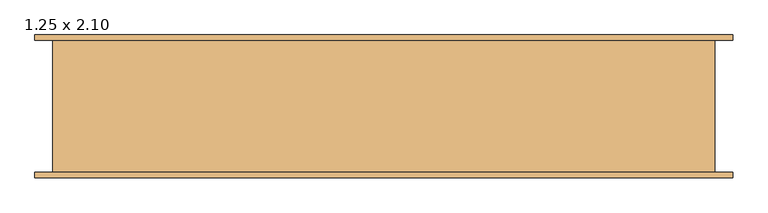
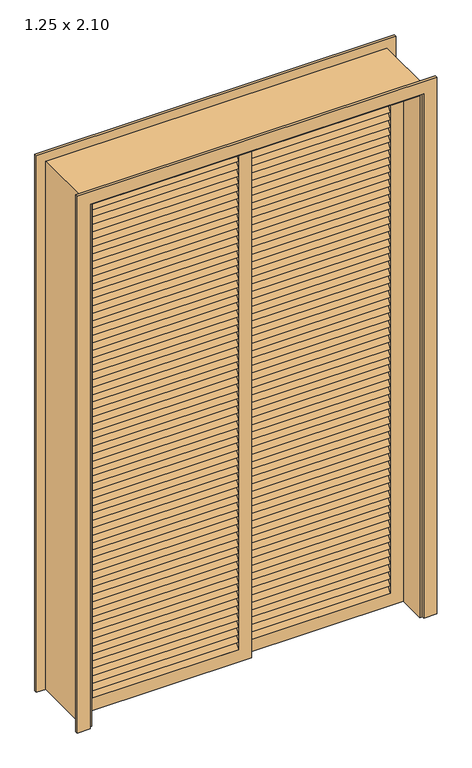
"""IFC4 building model written with IfcOpenShell, lengths in millimetres: door geometry, .CC_ND 300_PORTA DE CORRER_3 FOLHAS_VENEZIANA_VIDRO_COM EXTENSÃO : 1.25 x 2.10."""

import ifcopenshell
import ifcopenshell.guid

model = None  # the IFC model being written
_history = None  # IfcOwnerHistory: only IFC2X3 demands one
_inside = {}  # id of a spatial element -> (the spatial element, [elements in it])
_under = {}  # id of a project, library or spatial element -> (it, [spatial elements below it])
_declared = {}  # id of a project -> (the project, [libraries it declares])
_typed = {}  # id of a type object -> (the type object, [elements of that type])
_made_of = {}  # id of a material, layer set ... -> (it, [elements and type objects made of it])


def new_model(schema):
    """Start an empty IFC model of exactly this schema.

    Asked for "IFC4X3", IfcOpenShell would pick the latest addendum, in which some entities
    have other attributes; the version numbers below select the first issue.
    IFC2X3 requires an IfcOwnerHistory on every rooted entity: one is made here for all.
    """
    global model, _history
    if schema == "IFC4X3":
        model = ifcopenshell.file(schema_version=(4, 3, 0, 0))
    else:
        model = ifcopenshell.file(schema=schema)
    _inside.clear()
    _under.clear()
    _declared.clear()
    _typed.clear()
    _made_of.clear()
    _history = None
    if model.schema == "IFC2X3":
        org = make("IfcOrganization", Name="unknown")
        user = make(
            "IfcPersonAndOrganization",
            ThePerson=make("IfcPerson", FamilyName="unknown"),
            TheOrganization=org,
        )
        app = make(
            "IfcApplication",
            ApplicationDeveloper=org,
            Version="unknown",
            ApplicationFullName="unknown",
            ApplicationIdentifier="unknown",
        )
        _history = make(
            "IfcOwnerHistory",
            OwningUser=user,
            OwningApplication=app,
            ChangeAction="ADDED",
            CreationDate=0,
        )
    return model


def make(cls, **values):
    """One entity of the class cls with the attributes given. An attribute that is None is left unset."""
    return model.create_entity(
        cls, **{name: value for name, value in values.items() if value is not None}
    )


def rooted(cls, **values):
    """An entity with a GlobalId (a new one), such as an element, a storey or a relation."""
    return make(cls, GlobalId=ifcopenshell.guid.new(), OwnerHistory=_history, **values)


def si_unit(unit_type, name, prefix=None):
    """IfcSIUnit, for example si_unit("LENGTHUNIT", "METRE", prefix="MILLI")."""
    return make("IfcSIUnit", UnitType=unit_type, Prefix=prefix, Name=name)


def assignment(units):
    """IfcUnitAssignment: the units of a project."""
    return None if units is None else make("IfcUnitAssignment", Units=units)


def point(xyz):
    """IfcCartesianPoint."""
    return None if xyz is None else make("IfcCartesianPoint", Coordinates=xyz)


def direction(xyz):
    """IfcDirection."""
    return None if xyz is None else make("IfcDirection", DirectionRatios=xyz)


def frame(location, z_axis=None, x_axis=None):
    """IfcAxis2Placement3D, a coordinate frame: its origin and axes. An axis left out is left unset."""
    return make(
        "IfcAxis2Placement3D",
        Location=point(location),
        Axis=direction(z_axis),
        RefDirection=direction(x_axis),
    )


def origin():
    """The frame at (0, 0, 0) with its axes left unset."""
    return frame((0.0, 0.0, 0.0))


def place(relative_to, where):
    """IfcLocalPlacement: puts the frame where relative to a parent placement (None: the world)."""
    return make(
        "IfcLocalPlacement", PlacementRelTo=relative_to, RelativePlacement=where
    )


def context(
    kind, dimensions, precision=None, world=None, true_north=None, identifier=None
):
    """IfcGeometricRepresentationContext, for example the 3D "Model" context."""
    return make(
        "IfcGeometricRepresentationContext",
        ContextIdentifier=identifier,
        ContextType=kind,
        CoordinateSpaceDimension=dimensions,
        Precision=precision,
        WorldCoordinateSystem=world,
        TrueNorth=true_north,
    )


def project(units=None, contexts=None):
    """IfcProject with its units and contexts."""
    return rooted(
        "IfcProject",
        Name="project",
        RepresentationContexts=contexts,
        UnitsInContext=assignment(units),
    )


def spatial(cls, under=None, at=None, **own):
    """A site, building, storey or space (cls), placed at a placement, below another one or the project."""
    s = rooted(cls, ObjectPlacement=at, **own)
    if under is not None:
        _under.setdefault(under.id(), (under, []))[1].append(s)
    return s


def polyline(points):
    """IfcPolyline through the points."""
    return make("IfcPolyline", Points=[point(p) for p in points])


def outline(outer, holes=None, kind="AREA"):
    """IfcArbitraryClosedProfileDef: a profile drawn as a closed curve; with holes, ...WithVoids."""
    if holes is None:
        return make("IfcArbitraryClosedProfileDef", ProfileType=kind, OuterCurve=outer)
    return make(
        "IfcArbitraryProfileDefWithVoids",
        ProfileType=kind,
        OuterCurve=outer,
        InnerCurves=holes,
    )


def extrude(swept, where, along, depth):
    """IfcExtrudedAreaSolid: the profile swept, set in the frame where, extruded along a direction by depth."""
    return make(
        "IfcExtrudedAreaSolid",
        SweptArea=swept,
        Position=where,
        ExtrudedDirection=direction(along),
        Depth=depth,
    )


def shape(context_of_items, identifier, shape_type, items):
    """IfcShapeRepresentation: the items that make up one representation, for example the "Body"."""
    return make(
        "IfcShapeRepresentation",
        ContextOfItems=context_of_items,
        RepresentationIdentifier=identifier,
        RepresentationType=shape_type,
        Items=items,
    )


def source(mapping_origin, context_of_items, identifier, shape_type, items):
    """IfcRepresentationMap: a shape defined once, which mapped items show again and again."""
    return make(
        "IfcRepresentationMap",
        MappingOrigin=mapping_origin,
        MappedRepresentation=shape(context_of_items, identifier, shape_type, items),
    )


def transform(
    local_origin,
    x_axis=None,
    y_axis=None,
    z_axis=None,
    scale=None,
    scale2=None,
    scale3=None,
    uniform=True,
):
    """IfcCartesianTransformationOperator3D, or its non-uniform kind. x_axis, y_axis, z_axis: its Axis1, 2, 3."""
    if uniform:
        return make(
            "IfcCartesianTransformationOperator3D",
            Axis1=direction(x_axis),
            Axis2=direction(y_axis),
            LocalOrigin=point(local_origin),
            Scale=scale,
            Axis3=direction(z_axis),
        )
    return make(
        "IfcCartesianTransformationOperator3DnonUniform",
        Axis1=direction(x_axis),
        Axis2=direction(y_axis),
        LocalOrigin=point(local_origin),
        Scale=scale,
        Axis3=direction(z_axis),
        Scale2=scale2,
        Scale3=scale3,
    )


def mapped(mapping_source, mapping_target):
    """IfcMappedItem: shows the shape of a source again, moved by a transform."""
    return make(
        "IfcMappedItem", MappingSource=mapping_source, MappingTarget=mapping_target
    )


def made_of(thing, what):
    """Note that an element or type object is made of a material, layer set ...; save() writes the relation."""
    if what is not None:
        _made_of.setdefault(what.id(), (what, []))[1].append(thing)
    return thing


def element(
    cls,
    number,
    at=None,
    inside=None,
    cuts=None,
    type_object=None,
    material=None,
    context=None,
    identifier="Body",
    shape_type=None,
    held_by="IfcProductDefinitionShape",
    body=None,
    shapes=None,
    **own,
):
    """One element of the class cls, such as IfcWall. Its Tag is "e" and its number.

    at: its placement. inside: the storey or other place that contains it. cuts: it is an
    opening in that element (IfcRelVoidsElement). A single representation is given by context,
    identifier, shape_type and body (its items); several are given by shapes. held_by: the class
    of the entity that holds the representations. save() writes the other relations.
    """
    e = rooted(cls, Tag="e%d" % number, ObjectPlacement=at, **own)
    if body is not None:
        shapes = [shape(context, identifier, shape_type, body)]
    if shapes is not None:
        e.Representation = make(held_by, Representations=shapes)
    if inside is not None:
        _inside.setdefault(inside.id(), (inside, []))[1].append(e)
    if cuts is not None:
        rooted(
            "IfcRelVoidsElement", RelatingBuildingElement=cuts, RelatedOpeningElement=e
        )
    if type_object is not None:
        _typed.setdefault(type_object.id(), (type_object, []))[1].append(e)
    return made_of(e, material)


def aggregate(whole, parts):
    """IfcRelAggregates: a whole, such as a stair, and the parts it consists of."""
    return rooted("IfcRelAggregates", RelatingObject=whole, RelatedObjects=parts)


def save(model, path):
    """Write the relations noted so far, then the file.

    IfcRelAggregates (storeys below a building ...), IfcRelContainedInSpatialStructure (elements
    in a storey), IfcRelDefinesByType, IfcRelAssociatesMaterial and IfcRelDeclares: one each for
    every whole, place, type object, material and project.
    """
    for whole, parts in _under.values():
        aggregate(whole, parts)
    for where, things in _inside.values():
        rooted(
            "IfcRelContainedInSpatialStructure",
            RelatedElements=things,
            RelatingStructure=where,
        )
    for kind, things in _typed.values():
        rooted("IfcRelDefinesByType", RelatedObjects=things, RelatingType=kind)
    for what, things in _made_of.values():
        rooted("IfcRelAssociatesMaterial", RelatedObjects=things, RelatingMaterial=what)
    for by, libraries in _declared.values():
        rooted("IfcRelDeclares", RelatingContext=by, RelatedDefinitions=libraries)
    model.write(path)


def door_1_25_x_2_10_052434fb(model_context):
    return source(origin(), model_context, "Body", "SweptSolid", [
        extrude(outline(polyline([(575.0, 26.0), (20.0, 26.0), (20.0, 34.0), (575.0, 34.0), (575.0, 26.0)])), frame((0.0, 0.0, 50.0), z_axis=(0.0, 0.0, 1.0), x_axis=(1.0, 0.0, 0.0)), (0.0, 0.0, 1.0), 2000.0),
        extrude(outline(polyline([(2100.0, 625.0), (2100.0, -30.0), (0.0, -30.0), (0.0, 625.0), (2100.0, 625.0)]), holes=[polyline([(2050.0, 575.0), (50.0, 575.0), (50.0, 20.0), (2050.0, 20.0), (2050.0, 575.0)])]), frame((0.0, 15.0, 0.0), z_axis=(0.0, 1.0, 0.0), x_axis=(0.0, 0.0, 1.0)), (0.0, 0.0, 1.0), 30.0),
        extrude(outline(polyline([(-40.0, 1985.2272727), (-45.0, 1985.2272727), (-20.0, 2020.2272727), (-15.0, 2020.2272727), (-40.0, 1985.2272727)])), frame((-575.0, 0.0, 0.0), z_axis=(1.0, 0.0, 0.0), x_axis=(0.0, 1.0, 0.0)), (0.0, 0.0, 1.0), 555.0),
        extrude(outline(polyline([(-40.0, 1955.4545455), (-45.0, 1955.4545455), (-20.0, 1990.4545455), (-15.0, 1990.4545455), (-40.0, 1955.4545455)])), frame((-575.0, 0.0, 0.0), z_axis=(1.0, 0.0, 0.0), x_axis=(0.0, 1.0, 0.0)), (0.0, 0.0, 1.0), 555.0),
        extrude(outline(polyline([(-40.0, 1925.6818182), (-45.0, 1925.6818182), (-20.0, 1960.6818182), (-15.0, 1960.6818182), (-40.0, 1925.6818182)])), frame((-575.0, 0.0, 0.0), z_axis=(1.0, 0.0, 0.0), x_axis=(0.0, 1.0, 0.0)), (0.0, 0.0, 1.0), 555.0),
        extrude(outline(polyline([(-40.0, 1895.9090909), (-45.0, 1895.9090909), (-20.0, 1930.9090909), (-15.0, 1930.9090909), (-40.0, 1895.9090909)])), frame((-575.0, 0.0, 0.0), z_axis=(1.0, 0.0, 0.0), x_axis=(0.0, 1.0, 0.0)), (0.0, 0.0, 1.0), 555.0),
        extrude(outline(polyline([(-40.0, 1866.1363636), (-45.0, 1866.1363636), (-20.0, 1901.1363636), (-15.0, 1901.1363636), (-40.0, 1866.1363636)])), frame((-575.0, 0.0, 0.0), z_axis=(1.0, 0.0, 0.0), x_axis=(0.0, 1.0, 0.0)), (0.0, 0.0, 1.0), 555.0),
        extrude(outline(polyline([(-40.0, 1836.3636364), (-45.0, 1836.3636364), (-20.0, 1871.3636364), (-15.0, 1871.3636364), (-40.0, 1836.3636364)])), frame((-575.0, 0.0, 0.0), z_axis=(1.0, 0.0, 0.0), x_axis=(0.0, 1.0, 0.0)), (0.0, 0.0, 1.0), 555.0),
        extrude(outline(polyline([(-40.0, 1806.5909091), (-45.0, 1806.5909091), (-20.0, 1841.5909091), (-15.0, 1841.5909091), (-40.0, 1806.5909091)])), frame((-575.0, 0.0, 0.0), z_axis=(1.0, 0.0, 0.0), x_axis=(0.0, 1.0, 0.0)), (0.0, 0.0, 1.0), 555.0),
        extrude(outline(polyline([(-40.0, 1776.8181818), (-45.0, 1776.8181818), (-20.0, 1811.8181818), (-15.0, 1811.8181818), (-40.0, 1776.8181818)])), frame((-575.0, 0.0, 0.0), z_axis=(1.0, 0.0, 0.0), x_axis=(0.0, 1.0, 0.0)), (0.0, 0.0, 1.0), 555.0),
        extrude(outline(polyline([(-40.0, 1747.0454545), (-45.0, 1747.0454545), (-20.0, 1782.0454545), (-15.0, 1782.0454545), (-40.0, 1747.0454545)])), frame((-575.0, 0.0, 0.0), z_axis=(1.0, 0.0, 0.0), x_axis=(0.0, 1.0, 0.0)), (0.0, 0.0, 1.0), 555.0),
        extrude(outline(polyline([(-40.0, 1717.2727273), (-45.0, 1717.2727273), (-20.0, 1752.2727273), (-15.0, 1752.2727273), (-40.0, 1717.2727273)])), frame((-575.0, 0.0, 0.0), z_axis=(1.0, 0.0, 0.0), x_axis=(0.0, 1.0, 0.0)), (0.0, 0.0, 1.0), 555.0),
        extrude(outline(polyline([(-40.0, 1687.5), (-45.0, 1687.5), (-20.0, 1722.5), (-15.0, 1722.5), (-40.0, 1687.5)])), frame((-575.0, 0.0, 0.0), z_axis=(1.0, 0.0, 0.0), x_axis=(0.0, 1.0, 0.0)), (0.0, 0.0, 1.0), 555.0),
        extrude(outline(polyline([(-40.0, 1657.7272727), (-45.0, 1657.7272727), (-20.0, 1692.7272727), (-15.0, 1692.7272727), (-40.0, 1657.7272727)])), frame((-575.0, 0.0, 0.0), z_axis=(1.0, 0.0, 0.0), x_axis=(0.0, 1.0, 0.0)), (0.0, 0.0, 1.0), 555.0),
        extrude(outline(polyline([(-40.0, 1627.9545455), (-45.0, 1627.9545455), (-20.0, 1662.9545455), (-15.0, 1662.9545455), (-40.0, 1627.9545455)])), frame((-575.0, 0.0, 0.0), z_axis=(1.0, 0.0, 0.0), x_axis=(0.0, 1.0, 0.0)), (0.0, 0.0, 1.0), 555.0),
        extrude(outline(polyline([(-40.0, 1598.1818182), (-45.0, 1598.1818182), (-20.0, 1633.1818182), (-15.0, 1633.1818182), (-40.0, 1598.1818182)])), frame((-575.0, 0.0, 0.0), z_axis=(1.0, 0.0, 0.0), x_axis=(0.0, 1.0, 0.0)), (0.0, 0.0, 1.0), 555.0),
        extrude(outline(polyline([(-40.0, 1568.4090909), (-45.0, 1568.4090909), (-20.0, 1603.4090909), (-15.0, 1603.4090909), (-40.0, 1568.4090909)])), frame((-575.0, 0.0, 0.0), z_axis=(1.0, 0.0, 0.0), x_axis=(0.0, 1.0, 0.0)), (0.0, 0.0, 1.0), 555.0),
        extrude(outline(polyline([(-40.0, 1538.6363636), (-45.0, 1538.6363636), (-20.0, 1573.6363636), (-15.0, 1573.6363636), (-40.0, 1538.6363636)])), frame((-575.0, 0.0, 0.0), z_axis=(1.0, 0.0, 0.0), x_axis=(0.0, 1.0, 0.0)), (0.0, 0.0, 1.0), 555.0),
        extrude(outline(polyline([(-40.0, 1508.8636364), (-45.0, 1508.8636364), (-20.0, 1543.8636364), (-15.0, 1543.8636364), (-40.0, 1508.8636364)])), frame((-575.0, 0.0, 0.0), z_axis=(1.0, 0.0, 0.0), x_axis=(0.0, 1.0, 0.0)), (0.0, 0.0, 1.0), 555.0),
        extrude(outline(polyline([(-40.0, 1479.0909091), (-45.0, 1479.0909091), (-20.0, 1514.0909091), (-15.0, 1514.0909091), (-40.0, 1479.0909091)])), frame((-575.0, 0.0, 0.0), z_axis=(1.0, 0.0, 0.0), x_axis=(0.0, 1.0, 0.0)), (0.0, 0.0, 1.0), 555.0),
        extrude(outline(polyline([(-40.0, 1449.3181818), (-45.0, 1449.3181818), (-20.0, 1484.3181818), (-15.0, 1484.3181818), (-40.0, 1449.3181818)])), frame((-575.0, 0.0, 0.0), z_axis=(1.0, 0.0, 0.0), x_axis=(0.0, 1.0, 0.0)), (0.0, 0.0, 1.0), 555.0),
        extrude(outline(polyline([(-40.0, 1419.5454545), (-45.0, 1419.5454545), (-20.0, 1454.5454545), (-15.0, 1454.5454545), (-40.0, 1419.5454545)])), frame((-575.0, 0.0, 0.0), z_axis=(1.0, 0.0, 0.0), x_axis=(0.0, 1.0, 0.0)), (0.0, 0.0, 1.0), 555.0),
        extrude(outline(polyline([(-40.0, 1389.7727273), (-45.0, 1389.7727273), (-20.0, 1424.7727273), (-15.0, 1424.7727273), (-40.0, 1389.7727273)])), frame((-575.0, 0.0, 0.0), z_axis=(1.0, 0.0, 0.0), x_axis=(0.0, 1.0, 0.0)), (0.0, 0.0, 1.0), 555.0),
        extrude(outline(polyline([(-40.0, 1360.0), (-45.0, 1360.0), (-20.0, 1395.0), (-15.0, 1395.0), (-40.0, 1360.0)])), frame((-575.0, 0.0, 0.0), z_axis=(1.0, 0.0, 0.0), x_axis=(0.0, 1.0, 0.0)), (0.0, 0.0, 1.0), 555.0),
        extrude(outline(polyline([(-40.0, 1330.2272727), (-45.0, 1330.2272727), (-20.0, 1365.2272727), (-15.0, 1365.2272727), (-40.0, 1330.2272727)])), frame((-575.0, 0.0, 0.0), z_axis=(1.0, 0.0, 0.0), x_axis=(0.0, 1.0, 0.0)), (0.0, 0.0, 1.0), 555.0),
        extrude(outline(polyline([(-40.0, 1300.4545455), (-45.0, 1300.4545455), (-20.0, 1335.4545455), (-15.0, 1335.4545455), (-40.0, 1300.4545455)])), frame((-575.0, 0.0, 0.0), z_axis=(1.0, 0.0, 0.0), x_axis=(0.0, 1.0, 0.0)), (0.0, 0.0, 1.0), 555.0),
        extrude(outline(polyline([(-40.0, 1270.6818182), (-45.0, 1270.6818182), (-20.0, 1305.6818182), (-15.0, 1305.6818182), (-40.0, 1270.6818182)])), frame((-575.0, 0.0, 0.0), z_axis=(1.0, 0.0, 0.0), x_axis=(0.0, 1.0, 0.0)), (0.0, 0.0, 1.0), 555.0),
        extrude(outline(polyline([(-40.0, 1240.9090909), (-45.0, 1240.9090909), (-20.0, 1275.9090909), (-15.0, 1275.9090909), (-40.0, 1240.9090909)])), frame((-575.0, 0.0, 0.0), z_axis=(1.0, 0.0, 0.0), x_axis=(0.0, 1.0, 0.0)), (0.0, 0.0, 1.0), 555.0),
        extrude(outline(polyline([(-40.0, 1211.1363636), (-45.0, 1211.1363636), (-20.0, 1246.1363636), (-15.0, 1246.1363636), (-40.0, 1211.1363636)])), frame((-575.0, 0.0, 0.0), z_axis=(1.0, 0.0, 0.0), x_axis=(0.0, 1.0, 0.0)), (0.0, 0.0, 1.0), 555.0),
        extrude(outline(polyline([(-40.0, 1181.3636364), (-45.0, 1181.3636364), (-20.0, 1216.3636364), (-15.0, 1216.3636364), (-40.0, 1181.3636364)])), frame((-575.0, 0.0, 0.0), z_axis=(1.0, 0.0, 0.0), x_axis=(0.0, 1.0, 0.0)), (0.0, 0.0, 1.0), 555.0),
        extrude(outline(polyline([(-40.0, 1151.5909091), (-45.0, 1151.5909091), (-20.0, 1186.5909091), (-15.0, 1186.5909091), (-40.0, 1151.5909091)])), frame((-575.0, 0.0, 0.0), z_axis=(1.0, 0.0, 0.0), x_axis=(0.0, 1.0, 0.0)), (0.0, 0.0, 1.0), 555.0),
        extrude(outline(polyline([(-40.0, 1121.8181818), (-45.0, 1121.8181818), (-20.0, 1156.8181818), (-15.0, 1156.8181818), (-40.0, 1121.8181818)])), frame((-575.0, 0.0, 0.0), z_axis=(1.0, 0.0, 0.0), x_axis=(0.0, 1.0, 0.0)), (0.0, 0.0, 1.0), 555.0),
        extrude(outline(polyline([(-40.0, 1092.0454545), (-45.0, 1092.0454545), (-20.0, 1127.0454545), (-15.0, 1127.0454545), (-40.0, 1092.0454545)])), frame((-575.0, 0.0, 0.0), z_axis=(1.0, 0.0, 0.0), x_axis=(0.0, 1.0, 0.0)), (0.0, 0.0, 1.0), 555.0),
        extrude(outline(polyline([(-40.0, 1062.2727273), (-45.0, 1062.2727273), (-20.0, 1097.2727273), (-15.0, 1097.2727273), (-40.0, 1062.2727273)])), frame((-575.0, 0.0, 0.0), z_axis=(1.0, 0.0, 0.0), x_axis=(0.0, 1.0, 0.0)), (0.0, 0.0, 1.0), 555.0),
        extrude(outline(polyline([(-40.0, 1032.5), (-45.0, 1032.5), (-20.0, 1067.5), (-15.0, 1067.5), (-40.0, 1032.5)])), frame((-575.0, 0.0, 0.0), z_axis=(1.0, 0.0, 0.0), x_axis=(0.0, 1.0, 0.0)), (0.0, 0.0, 1.0), 555.0),
        extrude(outline(polyline([(-40.0, 1002.7272727), (-45.0, 1002.7272727), (-20.0, 1037.7272727), (-15.0, 1037.7272727), (-40.0, 1002.7272727)])), frame((-575.0, 0.0, 0.0), z_axis=(1.0, 0.0, 0.0), x_axis=(0.0, 1.0, 0.0)), (0.0, 0.0, 1.0), 555.0),
        extrude(outline(polyline([(-40.0, 972.9545455), (-45.0, 972.9545455), (-20.0, 1007.9545455), (-15.0, 1007.9545455), (-40.0, 972.9545455)])), frame((-575.0, 0.0, 0.0), z_axis=(1.0, 0.0, 0.0), x_axis=(0.0, 1.0, 0.0)), (0.0, 0.0, 1.0), 555.0),
        extrude(outline(polyline([(-40.0, 943.1818182), (-45.0, 943.1818182), (-20.0, 978.1818182), (-15.0, 978.1818182), (-40.0, 943.1818182)])), frame((-575.0, 0.0, 0.0), z_axis=(1.0, 0.0, 0.0), x_axis=(0.0, 1.0, 0.0)), (0.0, 0.0, 1.0), 555.0),
        extrude(outline(polyline([(-40.0, 913.4090909), (-45.0, 913.4090909), (-20.0, 948.4090909), (-15.0, 948.4090909), (-40.0, 913.4090909)])), frame((-575.0, 0.0, 0.0), z_axis=(1.0, 0.0, 0.0), x_axis=(0.0, 1.0, 0.0)), (0.0, 0.0, 1.0), 555.0),
        extrude(outline(polyline([(-40.0, 883.6363636), (-45.0, 883.6363636), (-20.0, 918.6363636), (-15.0, 918.6363636), (-40.0, 883.6363636)])), frame((-575.0, 0.0, 0.0), z_axis=(1.0, 0.0, 0.0), x_axis=(0.0, 1.0, 0.0)), (0.0, 0.0, 1.0), 555.0),
        extrude(outline(polyline([(-40.0, 853.8636364), (-45.0, 853.8636364), (-20.0, 888.8636364), (-15.0, 888.8636364), (-40.0, 853.8636364)])), frame((-575.0, 0.0, 0.0), z_axis=(1.0, 0.0, 0.0), x_axis=(0.0, 1.0, 0.0)), (0.0, 0.0, 1.0), 555.0),
        extrude(outline(polyline([(-40.0, 824.0909091), (-45.0, 824.0909091), (-20.0, 859.0909091), (-15.0, 859.0909091), (-40.0, 824.0909091)])), frame((-575.0, 0.0, 0.0), z_axis=(1.0, 0.0, 0.0), x_axis=(0.0, 1.0, 0.0)), (0.0, 0.0, 1.0), 555.0),
        extrude(outline(polyline([(-40.0, 794.3181818), (-45.0, 794.3181818), (-20.0, 829.3181818), (-15.0, 829.3181818), (-40.0, 794.3181818)])), frame((-575.0, 0.0, 0.0), z_axis=(1.0, 0.0, 0.0), x_axis=(0.0, 1.0, 0.0)), (0.0, 0.0, 1.0), 555.0),
        extrude(outline(polyline([(-40.0, 764.5454545), (-45.0, 764.5454545), (-20.0, 799.5454545), (-15.0, 799.5454545), (-40.0, 764.5454545)])), frame((-575.0, 0.0, 0.0), z_axis=(1.0, 0.0, 0.0), x_axis=(0.0, 1.0, 0.0)), (0.0, 0.0, 1.0), 555.0),
        extrude(outline(polyline([(-40.0, 734.7727273), (-45.0, 734.7727273), (-20.0, 769.7727273), (-15.0, 769.7727273), (-40.0, 734.7727273)])), frame((-575.0, 0.0, 0.0), z_axis=(1.0, 0.0, 0.0), x_axis=(0.0, 1.0, 0.0)), (0.0, 0.0, 1.0), 555.0),
        extrude(outline(polyline([(-40.0, 705.0), (-45.0, 705.0), (-20.0, 740.0), (-15.0, 740.0), (-40.0, 705.0)])), frame((-575.0, 0.0, 0.0), z_axis=(1.0, 0.0, 0.0), x_axis=(0.0, 1.0, 0.0)), (0.0, 0.0, 1.0), 555.0),
        extrude(outline(polyline([(-40.0, 675.2272727), (-45.0, 675.2272727), (-20.0, 710.2272727), (-15.0, 710.2272727), (-40.0, 675.2272727)])), frame((-575.0, 0.0, 0.0), z_axis=(1.0, 0.0, 0.0), x_axis=(0.0, 1.0, 0.0)), (0.0, 0.0, 1.0), 555.0),
        extrude(outline(polyline([(-40.0, 645.4545455), (-45.0, 645.4545455), (-20.0, 680.4545455), (-15.0, 680.4545455), (-40.0, 645.4545455)])), frame((-575.0, 0.0, 0.0), z_axis=(1.0, 0.0, 0.0), x_axis=(0.0, 1.0, 0.0)), (0.0, 0.0, 1.0), 555.0),
        extrude(outline(polyline([(-40.0, 615.6818182), (-45.0, 615.6818182), (-20.0, 650.6818182), (-15.0, 650.6818182), (-40.0, 615.6818182)])), frame((-575.0, 0.0, 0.0), z_axis=(1.0, 0.0, 0.0), x_axis=(0.0, 1.0, 0.0)), (0.0, 0.0, 1.0), 555.0),
        extrude(outline(polyline([(-40.0, 585.9090909), (-45.0, 585.9090909), (-20.0, 620.9090909), (-15.0, 620.9090909), (-40.0, 585.9090909)])), frame((-575.0, 0.0, 0.0), z_axis=(1.0, 0.0, 0.0), x_axis=(0.0, 1.0, 0.0)), (0.0, 0.0, 1.0), 555.0),
        extrude(outline(polyline([(-40.0, 556.1363636), (-45.0, 556.1363636), (-20.0, 591.1363636), (-15.0, 591.1363636), (-40.0, 556.1363636)])), frame((-575.0, 0.0, 0.0), z_axis=(1.0, 0.0, 0.0), x_axis=(0.0, 1.0, 0.0)), (0.0, 0.0, 1.0), 555.0),
        extrude(outline(polyline([(-40.0, 526.3636364), (-45.0, 526.3636364), (-20.0, 561.3636364), (-15.0, 561.3636364), (-40.0, 526.3636364)])), frame((-575.0, 0.0, 0.0), z_axis=(1.0, 0.0, 0.0), x_axis=(0.0, 1.0, 0.0)), (0.0, 0.0, 1.0), 555.0),
        extrude(outline(polyline([(-40.0, 496.5909091), (-45.0, 496.5909091), (-20.0, 531.5909091), (-15.0, 531.5909091), (-40.0, 496.5909091)])), frame((-575.0, 0.0, 0.0), z_axis=(1.0, 0.0, 0.0), x_axis=(0.0, 1.0, 0.0)), (0.0, 0.0, 1.0), 555.0),
        extrude(outline(polyline([(-40.0, 466.8181818), (-45.0, 466.8181818), (-20.0, 501.8181818), (-15.0, 501.8181818), (-40.0, 466.8181818)])), frame((-575.0, 0.0, 0.0), z_axis=(1.0, 0.0, 0.0), x_axis=(0.0, 1.0, 0.0)), (0.0, 0.0, 1.0), 555.0),
        extrude(outline(polyline([(-40.0, 437.0454545), (-45.0, 437.0454545), (-20.0, 472.0454545), (-15.0, 472.0454545), (-40.0, 437.0454545)])), frame((-575.0, 0.0, 0.0), z_axis=(1.0, 0.0, 0.0), x_axis=(0.0, 1.0, 0.0)), (0.0, 0.0, 1.0), 555.0),
        extrude(outline(polyline([(-40.0, 407.2727273), (-45.0, 407.2727273), (-20.0, 442.2727273), (-15.0, 442.2727273), (-40.0, 407.2727273)])), frame((-575.0, 0.0, 0.0), z_axis=(1.0, 0.0, 0.0), x_axis=(0.0, 1.0, 0.0)), (0.0, 0.0, 1.0), 555.0),
        extrude(outline(polyline([(-40.0, 377.5), (-45.0, 377.5), (-20.0, 412.5), (-15.0, 412.5), (-40.0, 377.5)])), frame((-575.0, 0.0, 0.0), z_axis=(1.0, 0.0, 0.0), x_axis=(0.0, 1.0, 0.0)), (0.0, 0.0, 1.0), 555.0),
        extrude(outline(polyline([(-40.0, 347.7272727), (-45.0, 347.7272727), (-20.0, 382.7272727), (-15.0, 382.7272727), (-40.0, 347.7272727)])), frame((-575.0, 0.0, 0.0), z_axis=(1.0, 0.0, 0.0), x_axis=(0.0, 1.0, 0.0)), (0.0, 0.0, 1.0), 555.0),
        extrude(outline(polyline([(-40.0, 317.9545455), (-45.0, 317.9545455), (-20.0, 352.9545455), (-15.0, 352.9545455), (-40.0, 317.9545455)])), frame((-575.0, 0.0, 0.0), z_axis=(1.0, 0.0, 0.0), x_axis=(0.0, 1.0, 0.0)), (0.0, 0.0, 1.0), 555.0),
        extrude(outline(polyline([(-40.0, 288.1818182), (-45.0, 288.1818182), (-20.0, 323.1818182), (-15.0, 323.1818182), (-40.0, 288.1818182)])), frame((-575.0, 0.0, 0.0), z_axis=(1.0, 0.0, 0.0), x_axis=(0.0, 1.0, 0.0)), (0.0, 0.0, 1.0), 555.0),
        extrude(outline(polyline([(-40.0, 258.4090909), (-45.0, 258.4090909), (-20.0, 293.4090909), (-15.0, 293.4090909), (-40.0, 258.4090909)])), frame((-575.0, 0.0, 0.0), z_axis=(1.0, 0.0, 0.0), x_axis=(0.0, 1.0, 0.0)), (0.0, 0.0, 1.0), 555.0),
        extrude(outline(polyline([(-40.0, 228.6363636), (-45.0, 228.6363636), (-20.0, 263.6363636), (-15.0, 263.6363636), (-40.0, 228.6363636)])), frame((-575.0, 0.0, 0.0), z_axis=(1.0, 0.0, 0.0), x_axis=(0.0, 1.0, 0.0)), (0.0, 0.0, 1.0), 555.0),
        extrude(outline(polyline([(-40.0, 198.8636364), (-45.0, 198.8636364), (-20.0, 233.8636364), (-15.0, 233.8636364), (-40.0, 198.8636364)])), frame((-575.0, 0.0, 0.0), z_axis=(1.0, 0.0, 0.0), x_axis=(0.0, 1.0, 0.0)), (0.0, 0.0, 1.0), 555.0),
        extrude(outline(polyline([(-40.0, 169.0909091), (-45.0, 169.0909091), (-20.0, 204.0909091), (-15.0, 204.0909091), (-40.0, 169.0909091)])), frame((-575.0, 0.0, 0.0), z_axis=(1.0, 0.0, 0.0), x_axis=(0.0, 1.0, 0.0)), (0.0, 0.0, 1.0), 555.0),
        extrude(outline(polyline([(-40.0, 139.3181818), (-45.0, 139.3181818), (-20.0, 174.3181818), (-15.0, 174.3181818), (-40.0, 139.3181818)])), frame((-575.0, 0.0, 0.0), z_axis=(1.0, 0.0, 0.0), x_axis=(0.0, 1.0, 0.0)), (0.0, 0.0, 1.0), 555.0),
        extrude(outline(polyline([(-40.0, 109.5454545), (-45.0, 109.5454545), (-20.0, 144.5454545), (-15.0, 144.5454545), (-40.0, 109.5454545)])), frame((-575.0, 0.0, 0.0), z_axis=(1.0, 0.0, 0.0), x_axis=(0.0, 1.0, 0.0)), (0.0, 0.0, 1.0), 555.0),
        extrude(outline(polyline([(-40.0, 79.7727273), (-45.0, 79.7727273), (-20.0, 114.7727273), (-15.0, 114.7727273), (-40.0, 79.7727273)])), frame((-575.0, 0.0, 0.0), z_axis=(1.0, 0.0, 0.0), x_axis=(0.0, 1.0, 0.0)), (0.0, 0.0, 1.0), 555.0),
        extrude(outline(polyline([(-40.0, 2015.0), (-45.0, 2015.0), (-20.0, 2050.0), (-15.0, 2050.0), (-40.0, 2015.0)])), frame((-575.0, 0.0, 0.0), z_axis=(1.0, 0.0, 0.0), x_axis=(0.0, 1.0, 0.0)), (0.0, 0.0, 1.0), 555.0),
        extrude(outline(polyline([(-40.0, 50.0), (-45.0, 50.0), (-20.0, 85.0), (-15.0, 85.0), (-40.0, 50.0)])), frame((-575.0, 0.0, 0.0), z_axis=(1.0, 0.0, 0.0), x_axis=(0.0, 1.0, 0.0)), (0.0, 0.0, 1.0), 555.0),
        extrude(outline(polyline([(2100.0, 30.0), (2100.0, -625.0), (0.0, -625.0), (0.0, 30.0), (2100.0, 30.0)]), holes=[polyline([(2050.0, -20.0), (50.0, -20.0), (50.0, -575.0), (2050.0, -575.0), (2050.0, -20.0)])]), frame((0.0, -45.0, 0.0), z_axis=(0.0, 1.0, 0.0), x_axis=(0.0, 0.0, 1.0)), (0.0, 0.0, 1.0), 30.0),
        extrude(outline(polyline([(-10.0, 1985.2272727), (-15.0, 1985.2272727), (10.0, 2020.2272727), (15.0, 2020.2272727), (-10.0, 1985.2272727)])), frame((20.0, 0.0, 0.0), z_axis=(1.0, 0.0, 0.0), x_axis=(0.0, 1.0, 0.0)), (0.0, 0.0, 1.0), 555.0),
        extrude(outline(polyline([(-10.0, 1955.4545455), (-15.0, 1955.4545455), (10.0, 1990.4545455), (15.0, 1990.4545455), (-10.0, 1955.4545455)])), frame((20.0, 0.0, 0.0), z_axis=(1.0, 0.0, 0.0), x_axis=(0.0, 1.0, 0.0)), (0.0, 0.0, 1.0), 555.0),
        extrude(outline(polyline([(-10.0, 1925.6818182), (-15.0, 1925.6818182), (10.0, 1960.6818182), (15.0, 1960.6818182), (-10.0, 1925.6818182)])), frame((20.0, 0.0, 0.0), z_axis=(1.0, 0.0, 0.0), x_axis=(0.0, 1.0, 0.0)), (0.0, 0.0, 1.0), 555.0),
        extrude(outline(polyline([(-10.0, 1895.9090909), (-15.0, 1895.9090909), (10.0, 1930.9090909), (15.0, 1930.9090909), (-10.0, 1895.9090909)])), frame((20.0, 0.0, 0.0), z_axis=(1.0, 0.0, 0.0), x_axis=(0.0, 1.0, 0.0)), (0.0, 0.0, 1.0), 555.0),
        extrude(outline(polyline([(-10.0, 1866.1363636), (-15.0, 1866.1363636), (10.0, 1901.1363636), (15.0, 1901.1363636), (-10.0, 1866.1363636)])), frame((20.0, 0.0, 0.0), z_axis=(1.0, 0.0, 0.0), x_axis=(0.0, 1.0, 0.0)), (0.0, 0.0, 1.0), 555.0),
        extrude(outline(polyline([(-10.0, 1836.3636364), (-15.0, 1836.3636364), (10.0, 1871.3636364), (15.0, 1871.3636364), (-10.0, 1836.3636364)])), frame((20.0, 0.0, 0.0), z_axis=(1.0, 0.0, 0.0), x_axis=(0.0, 1.0, 0.0)), (0.0, 0.0, 1.0), 555.0),
        extrude(outline(polyline([(-10.0, 1806.5909091), (-15.0, 1806.5909091), (10.0, 1841.5909091), (15.0, 1841.5909091), (-10.0, 1806.5909091)])), frame((20.0, 0.0, 0.0), z_axis=(1.0, 0.0, 0.0), x_axis=(0.0, 1.0, 0.0)), (0.0, 0.0, 1.0), 555.0),
        extrude(outline(polyline([(-10.0, 1776.8181818), (-15.0, 1776.8181818), (10.0, 1811.8181818), (15.0, 1811.8181818), (-10.0, 1776.8181818)])), frame((20.0, 0.0, 0.0), z_axis=(1.0, 0.0, 0.0), x_axis=(0.0, 1.0, 0.0)), (0.0, 0.0, 1.0), 555.0),
        extrude(outline(polyline([(-10.0, 1747.0454545), (-15.0, 1747.0454545), (10.0, 1782.0454545), (15.0, 1782.0454545), (-10.0, 1747.0454545)])), frame((20.0, 0.0, 0.0), z_axis=(1.0, 0.0, 0.0), x_axis=(0.0, 1.0, 0.0)), (0.0, 0.0, 1.0), 555.0),
        extrude(outline(polyline([(-10.0, 1717.2727273), (-15.0, 1717.2727273), (10.0, 1752.2727273), (15.0, 1752.2727273), (-10.0, 1717.2727273)])), frame((20.0, 0.0, 0.0), z_axis=(1.0, 0.0, 0.0), x_axis=(0.0, 1.0, 0.0)), (0.0, 0.0, 1.0), 555.0),
        extrude(outline(polyline([(-10.0, 1687.5), (-15.0, 1687.5), (10.0, 1722.5), (15.0, 1722.5), (-10.0, 1687.5)])), frame((20.0, 0.0, 0.0), z_axis=(1.0, 0.0, 0.0), x_axis=(0.0, 1.0, 0.0)), (0.0, 0.0, 1.0), 555.0),
        extrude(outline(polyline([(-10.0, 1657.7272727), (-15.0, 1657.7272727), (10.0, 1692.7272727), (15.0, 1692.7272727), (-10.0, 1657.7272727)])), frame((20.0, 0.0, 0.0), z_axis=(1.0, 0.0, 0.0), x_axis=(0.0, 1.0, 0.0)), (0.0, 0.0, 1.0), 555.0),
        extrude(outline(polyline([(-10.0, 1627.9545455), (-15.0, 1627.9545455), (10.0, 1662.9545455), (15.0, 1662.9545455), (-10.0, 1627.9545455)])), frame((20.0, 0.0, 0.0), z_axis=(1.0, 0.0, 0.0), x_axis=(0.0, 1.0, 0.0)), (0.0, 0.0, 1.0), 555.0),
        extrude(outline(polyline([(-10.0, 1598.1818182), (-15.0, 1598.1818182), (10.0, 1633.1818182), (15.0, 1633.1818182), (-10.0, 1598.1818182)])), frame((20.0, 0.0, 0.0), z_axis=(1.0, 0.0, 0.0), x_axis=(0.0, 1.0, 0.0)), (0.0, 0.0, 1.0), 555.0),
        extrude(outline(polyline([(-10.0, 1568.4090909), (-15.0, 1568.4090909), (10.0, 1603.4090909), (15.0, 1603.4090909), (-10.0, 1568.4090909)])), frame((20.0, 0.0, 0.0), z_axis=(1.0, 0.0, 0.0), x_axis=(0.0, 1.0, 0.0)), (0.0, 0.0, 1.0), 555.0),
        extrude(outline(polyline([(-10.0, 1538.6363636), (-15.0, 1538.6363636), (10.0, 1573.6363636), (15.0, 1573.6363636), (-10.0, 1538.6363636)])), frame((20.0, 0.0, 0.0), z_axis=(1.0, 0.0, 0.0), x_axis=(0.0, 1.0, 0.0)), (0.0, 0.0, 1.0), 555.0),
        extrude(outline(polyline([(-10.0, 1508.8636364), (-15.0, 1508.8636364), (10.0, 1543.8636364), (15.0, 1543.8636364), (-10.0, 1508.8636364)])), frame((20.0, 0.0, 0.0), z_axis=(1.0, 0.0, 0.0), x_axis=(0.0, 1.0, 0.0)), (0.0, 0.0, 1.0), 555.0),
        extrude(outline(polyline([(-10.0, 1479.0909091), (-15.0, 1479.0909091), (10.0, 1514.0909091), (15.0, 1514.0909091), (-10.0, 1479.0909091)])), frame((20.0, 0.0, 0.0), z_axis=(1.0, 0.0, 0.0), x_axis=(0.0, 1.0, 0.0)), (0.0, 0.0, 1.0), 555.0),
        extrude(outline(polyline([(-10.0, 1449.3181818), (-15.0, 1449.3181818), (10.0, 1484.3181818), (15.0, 1484.3181818), (-10.0, 1449.3181818)])), frame((20.0, 0.0, 0.0), z_axis=(1.0, 0.0, 0.0), x_axis=(0.0, 1.0, 0.0)), (0.0, 0.0, 1.0), 555.0),
        extrude(outline(polyline([(-10.0, 1419.5454545), (-15.0, 1419.5454545), (10.0, 1454.5454545), (15.0, 1454.5454545), (-10.0, 1419.5454545)])), frame((20.0, 0.0, 0.0), z_axis=(1.0, 0.0, 0.0), x_axis=(0.0, 1.0, 0.0)), (0.0, 0.0, 1.0), 555.0),
        extrude(outline(polyline([(-10.0, 1389.7727273), (-15.0, 1389.7727273), (10.0, 1424.7727273), (15.0, 1424.7727273), (-10.0, 1389.7727273)])), frame((20.0, 0.0, 0.0), z_axis=(1.0, 0.0, 0.0), x_axis=(0.0, 1.0, 0.0)), (0.0, 0.0, 1.0), 555.0),
        extrude(outline(polyline([(-10.0, 1360.0), (-15.0, 1360.0), (10.0, 1395.0), (15.0, 1395.0), (-10.0, 1360.0)])), frame((20.0, 0.0, 0.0), z_axis=(1.0, 0.0, 0.0), x_axis=(0.0, 1.0, 0.0)), (0.0, 0.0, 1.0), 555.0),
        extrude(outline(polyline([(-10.0, 1330.2272727), (-15.0, 1330.2272727), (10.0, 1365.2272727), (15.0, 1365.2272727), (-10.0, 1330.2272727)])), frame((20.0, 0.0, 0.0), z_axis=(1.0, 0.0, 0.0), x_axis=(0.0, 1.0, 0.0)), (0.0, 0.0, 1.0), 555.0),
        extrude(outline(polyline([(-10.0, 1300.4545455), (-15.0, 1300.4545455), (10.0, 1335.4545455), (15.0, 1335.4545455), (-10.0, 1300.4545455)])), frame((20.0, 0.0, 0.0), z_axis=(1.0, 0.0, 0.0), x_axis=(0.0, 1.0, 0.0)), (0.0, 0.0, 1.0), 555.0),
        extrude(outline(polyline([(-10.0, 1270.6818182), (-15.0, 1270.6818182), (10.0, 1305.6818182), (15.0, 1305.6818182), (-10.0, 1270.6818182)])), frame((20.0, 0.0, 0.0), z_axis=(1.0, 0.0, 0.0), x_axis=(0.0, 1.0, 0.0)), (0.0, 0.0, 1.0), 555.0),
        extrude(outline(polyline([(-10.0, 1240.9090909), (-15.0, 1240.9090909), (10.0, 1275.9090909), (15.0, 1275.9090909), (-10.0, 1240.9090909)])), frame((20.0, 0.0, 0.0), z_axis=(1.0, 0.0, 0.0), x_axis=(0.0, 1.0, 0.0)), (0.0, 0.0, 1.0), 555.0),
        extrude(outline(polyline([(-10.0, 1211.1363636), (-15.0, 1211.1363636), (10.0, 1246.1363636), (15.0, 1246.1363636), (-10.0, 1211.1363636)])), frame((20.0, 0.0, 0.0), z_axis=(1.0, 0.0, 0.0), x_axis=(0.0, 1.0, 0.0)), (0.0, 0.0, 1.0), 555.0),
        extrude(outline(polyline([(-10.0, 1181.3636364), (-15.0, 1181.3636364), (10.0, 1216.3636364), (15.0, 1216.3636364), (-10.0, 1181.3636364)])), frame((20.0, 0.0, 0.0), z_axis=(1.0, 0.0, 0.0), x_axis=(0.0, 1.0, 0.0)), (0.0, 0.0, 1.0), 555.0),
        extrude(outline(polyline([(-10.0, 1151.5909091), (-15.0, 1151.5909091), (10.0, 1186.5909091), (15.0, 1186.5909091), (-10.0, 1151.5909091)])), frame((20.0, 0.0, 0.0), z_axis=(1.0, 0.0, 0.0), x_axis=(0.0, 1.0, 0.0)), (0.0, 0.0, 1.0), 555.0),
        extrude(outline(polyline([(-10.0, 1121.8181818), (-15.0, 1121.8181818), (10.0, 1156.8181818), (15.0, 1156.8181818), (-10.0, 1121.8181818)])), frame((20.0, 0.0, 0.0), z_axis=(1.0, 0.0, 0.0), x_axis=(0.0, 1.0, 0.0)), (0.0, 0.0, 1.0), 555.0),
        extrude(outline(polyline([(-10.0, 1092.0454545), (-15.0, 1092.0454545), (10.0, 1127.0454545), (15.0, 1127.0454545), (-10.0, 1092.0454545)])), frame((20.0, 0.0, 0.0), z_axis=(1.0, 0.0, 0.0), x_axis=(0.0, 1.0, 0.0)), (0.0, 0.0, 1.0), 555.0),
        extrude(outline(polyline([(-10.0, 1062.2727273), (-15.0, 1062.2727273), (10.0, 1097.2727273), (15.0, 1097.2727273), (-10.0, 1062.2727273)])), frame((20.0, 0.0, 0.0), z_axis=(1.0, 0.0, 0.0), x_axis=(0.0, 1.0, 0.0)), (0.0, 0.0, 1.0), 555.0),
        extrude(outline(polyline([(-10.0, 1032.5), (-15.0, 1032.5), (10.0, 1067.5), (15.0, 1067.5), (-10.0, 1032.5)])), frame((20.0, 0.0, 0.0), z_axis=(1.0, 0.0, 0.0), x_axis=(0.0, 1.0, 0.0)), (0.0, 0.0, 1.0), 555.0),
        extrude(outline(polyline([(-10.0, 1002.7272727), (-15.0, 1002.7272727), (10.0, 1037.7272727), (15.0, 1037.7272727), (-10.0, 1002.7272727)])), frame((20.0, 0.0, 0.0), z_axis=(1.0, 0.0, 0.0), x_axis=(0.0, 1.0, 0.0)), (0.0, 0.0, 1.0), 555.0),
        extrude(outline(polyline([(-10.0, 972.9545455), (-15.0, 972.9545455), (10.0, 1007.9545455), (15.0, 1007.9545455), (-10.0, 972.9545455)])), frame((20.0, 0.0, 0.0), z_axis=(1.0, 0.0, 0.0), x_axis=(0.0, 1.0, 0.0)), (0.0, 0.0, 1.0), 555.0),
        extrude(outline(polyline([(-10.0, 943.1818182), (-15.0, 943.1818182), (10.0, 978.1818182), (15.0, 978.1818182), (-10.0, 943.1818182)])), frame((20.0, 0.0, 0.0), z_axis=(1.0, 0.0, 0.0), x_axis=(0.0, 1.0, 0.0)), (0.0, 0.0, 1.0), 555.0),
        extrude(outline(polyline([(-10.0, 913.4090909), (-15.0, 913.4090909), (10.0, 948.4090909), (15.0, 948.4090909), (-10.0, 913.4090909)])), frame((20.0, 0.0, 0.0), z_axis=(1.0, 0.0, 0.0), x_axis=(0.0, 1.0, 0.0)), (0.0, 0.0, 1.0), 555.0),
        extrude(outline(polyline([(-10.0, 883.6363636), (-15.0, 883.6363636), (10.0, 918.6363636), (15.0, 918.6363636), (-10.0, 883.6363636)])), frame((20.0, 0.0, 0.0), z_axis=(1.0, 0.0, 0.0), x_axis=(0.0, 1.0, 0.0)), (0.0, 0.0, 1.0), 555.0),
        extrude(outline(polyline([(-10.0, 853.8636364), (-15.0, 853.8636364), (10.0, 888.8636364), (15.0, 888.8636364), (-10.0, 853.8636364)])), frame((20.0, 0.0, 0.0), z_axis=(1.0, 0.0, 0.0), x_axis=(0.0, 1.0, 0.0)), (0.0, 0.0, 1.0), 555.0),
        extrude(outline(polyline([(-10.0, 824.0909091), (-15.0, 824.0909091), (10.0, 859.0909091), (15.0, 859.0909091), (-10.0, 824.0909091)])), frame((20.0, 0.0, 0.0), z_axis=(1.0, 0.0, 0.0), x_axis=(0.0, 1.0, 0.0)), (0.0, 0.0, 1.0), 555.0),
        extrude(outline(polyline([(-10.0, 794.3181818), (-15.0, 794.3181818), (10.0, 829.3181818), (15.0, 829.3181818), (-10.0, 794.3181818)])), frame((20.0, 0.0, 0.0), z_axis=(1.0, 0.0, 0.0), x_axis=(0.0, 1.0, 0.0)), (0.0, 0.0, 1.0), 555.0),
        extrude(outline(polyline([(-10.0, 764.5454545), (-15.0, 764.5454545), (10.0, 799.5454545), (15.0, 799.5454545), (-10.0, 764.5454545)])), frame((20.0, 0.0, 0.0), z_axis=(1.0, 0.0, 0.0), x_axis=(0.0, 1.0, 0.0)), (0.0, 0.0, 1.0), 555.0),
        extrude(outline(polyline([(-10.0, 734.7727273), (-15.0, 734.7727273), (10.0, 769.7727273), (15.0, 769.7727273), (-10.0, 734.7727273)])), frame((20.0, 0.0, 0.0), z_axis=(1.0, 0.0, 0.0), x_axis=(0.0, 1.0, 0.0)), (0.0, 0.0, 1.0), 555.0),
        extrude(outline(polyline([(-10.0, 705.0), (-15.0, 705.0), (10.0, 740.0), (15.0, 740.0), (-10.0, 705.0)])), frame((20.0, 0.0, 0.0), z_axis=(1.0, 0.0, 0.0), x_axis=(0.0, 1.0, 0.0)), (0.0, 0.0, 1.0), 555.0),
        extrude(outline(polyline([(-10.0, 675.2272727), (-15.0, 675.2272727), (10.0, 710.2272727), (15.0, 710.2272727), (-10.0, 675.2272727)])), frame((20.0, 0.0, 0.0), z_axis=(1.0, 0.0, 0.0), x_axis=(0.0, 1.0, 0.0)), (0.0, 0.0, 1.0), 555.0),
        extrude(outline(polyline([(-10.0, 645.4545455), (-15.0, 645.4545455), (10.0, 680.4545455), (15.0, 680.4545455), (-10.0, 645.4545455)])), frame((20.0, 0.0, 0.0), z_axis=(1.0, 0.0, 0.0), x_axis=(0.0, 1.0, 0.0)), (0.0, 0.0, 1.0), 555.0),
        extrude(outline(polyline([(-10.0, 615.6818182), (-15.0, 615.6818182), (10.0, 650.6818182), (15.0, 650.6818182), (-10.0, 615.6818182)])), frame((20.0, 0.0, 0.0), z_axis=(1.0, 0.0, 0.0), x_axis=(0.0, 1.0, 0.0)), (0.0, 0.0, 1.0), 555.0),
        extrude(outline(polyline([(-10.0, 585.9090909), (-15.0, 585.9090909), (10.0, 620.9090909), (15.0, 620.9090909), (-10.0, 585.9090909)])), frame((20.0, 0.0, 0.0), z_axis=(1.0, 0.0, 0.0), x_axis=(0.0, 1.0, 0.0)), (0.0, 0.0, 1.0), 555.0),
        extrude(outline(polyline([(-10.0, 556.1363636), (-15.0, 556.1363636), (10.0, 591.1363636), (15.0, 591.1363636), (-10.0, 556.1363636)])), frame((20.0, 0.0, 0.0), z_axis=(1.0, 0.0, 0.0), x_axis=(0.0, 1.0, 0.0)), (0.0, 0.0, 1.0), 555.0),
        extrude(outline(polyline([(-10.0, 526.3636364), (-15.0, 526.3636364), (10.0, 561.3636364), (15.0, 561.3636364), (-10.0, 526.3636364)])), frame((20.0, 0.0, 0.0), z_axis=(1.0, 0.0, 0.0), x_axis=(0.0, 1.0, 0.0)), (0.0, 0.0, 1.0), 555.0),
        extrude(outline(polyline([(-10.0, 496.5909091), (-15.0, 496.5909091), (10.0, 531.5909091), (15.0, 531.5909091), (-10.0, 496.5909091)])), frame((20.0, 0.0, 0.0), z_axis=(1.0, 0.0, 0.0), x_axis=(0.0, 1.0, 0.0)), (0.0, 0.0, 1.0), 555.0),
        extrude(outline(polyline([(-10.0, 466.8181818), (-15.0, 466.8181818), (10.0, 501.8181818), (15.0, 501.8181818), (-10.0, 466.8181818)])), frame((20.0, 0.0, 0.0), z_axis=(1.0, 0.0, 0.0), x_axis=(0.0, 1.0, 0.0)), (0.0, 0.0, 1.0), 555.0),
        extrude(outline(polyline([(-10.0, 437.0454545), (-15.0, 437.0454545), (10.0, 472.0454545), (15.0, 472.0454545), (-10.0, 437.0454545)])), frame((20.0, 0.0, 0.0), z_axis=(1.0, 0.0, 0.0), x_axis=(0.0, 1.0, 0.0)), (0.0, 0.0, 1.0), 555.0),
        extrude(outline(polyline([(-10.0, 407.2727273), (-15.0, 407.2727273), (10.0, 442.2727273), (15.0, 442.2727273), (-10.0, 407.2727273)])), frame((20.0, 0.0, 0.0), z_axis=(1.0, 0.0, 0.0), x_axis=(0.0, 1.0, 0.0)), (0.0, 0.0, 1.0), 555.0),
        extrude(outline(polyline([(-10.0, 377.5), (-15.0, 377.5), (10.0, 412.5), (15.0, 412.5), (-10.0, 377.5)])), frame((20.0, 0.0, 0.0), z_axis=(1.0, 0.0, 0.0), x_axis=(0.0, 1.0, 0.0)), (0.0, 0.0, 1.0), 555.0),
        extrude(outline(polyline([(-10.0, 347.7272727), (-15.0, 347.7272727), (10.0, 382.7272727), (15.0, 382.7272727), (-10.0, 347.7272727)])), frame((20.0, 0.0, 0.0), z_axis=(1.0, 0.0, 0.0), x_axis=(0.0, 1.0, 0.0)), (0.0, 0.0, 1.0), 555.0),
        extrude(outline(polyline([(-10.0, 317.9545455), (-15.0, 317.9545455), (10.0, 352.9545455), (15.0, 352.9545455), (-10.0, 317.9545455)])), frame((20.0, 0.0, 0.0), z_axis=(1.0, 0.0, 0.0), x_axis=(0.0, 1.0, 0.0)), (0.0, 0.0, 1.0), 555.0),
        extrude(outline(polyline([(-10.0, 288.1818182), (-15.0, 288.1818182), (10.0, 323.1818182), (15.0, 323.1818182), (-10.0, 288.1818182)])), frame((20.0, 0.0, 0.0), z_axis=(1.0, 0.0, 0.0), x_axis=(0.0, 1.0, 0.0)), (0.0, 0.0, 1.0), 555.0),
        extrude(outline(polyline([(-10.0, 258.4090909), (-15.0, 258.4090909), (10.0, 293.4090909), (15.0, 293.4090909), (-10.0, 258.4090909)])), frame((20.0, 0.0, 0.0), z_axis=(1.0, 0.0, 0.0), x_axis=(0.0, 1.0, 0.0)), (0.0, 0.0, 1.0), 555.0),
        extrude(outline(polyline([(-10.0, 228.6363636), (-15.0, 228.6363636), (10.0, 263.6363636), (15.0, 263.6363636), (-10.0, 228.6363636)])), frame((20.0, 0.0, 0.0), z_axis=(1.0, 0.0, 0.0), x_axis=(0.0, 1.0, 0.0)), (0.0, 0.0, 1.0), 555.0),
        extrude(outline(polyline([(-10.0, 198.8636364), (-15.0, 198.8636364), (10.0, 233.8636364), (15.0, 233.8636364), (-10.0, 198.8636364)])), frame((20.0, 0.0, 0.0), z_axis=(1.0, 0.0, 0.0), x_axis=(0.0, 1.0, 0.0)), (0.0, 0.0, 1.0), 555.0),
        extrude(outline(polyline([(-10.0, 169.0909091), (-15.0, 169.0909091), (10.0, 204.0909091), (15.0, 204.0909091), (-10.0, 169.0909091)])), frame((20.0, 0.0, 0.0), z_axis=(1.0, 0.0, 0.0), x_axis=(0.0, 1.0, 0.0)), (0.0, 0.0, 1.0), 555.0),
        extrude(outline(polyline([(-10.0, 139.3181818), (-15.0, 139.3181818), (10.0, 174.3181818), (15.0, 174.3181818), (-10.0, 139.3181818)])), frame((20.0, 0.0, 0.0), z_axis=(1.0, 0.0, 0.0), x_axis=(0.0, 1.0, 0.0)), (0.0, 0.0, 1.0), 555.0),
        extrude(outline(polyline([(-10.0, 109.5454545), (-15.0, 109.5454545), (10.0, 144.5454545), (15.0, 144.5454545), (-10.0, 109.5454545)])), frame((20.0, 0.0, 0.0), z_axis=(1.0, 0.0, 0.0), x_axis=(0.0, 1.0, 0.0)), (0.0, 0.0, 1.0), 555.0),
        extrude(outline(polyline([(-10.0, 79.7727273), (-15.0, 79.7727273), (10.0, 114.7727273), (15.0, 114.7727273), (-10.0, 79.7727273)])), frame((20.0, 0.0, 0.0), z_axis=(1.0, 0.0, 0.0), x_axis=(0.0, 1.0, 0.0)), (0.0, 0.0, 1.0), 555.0),
        extrude(outline(polyline([(-10.0, 2015.0), (-15.0, 2015.0), (10.0, 2050.0), (15.0, 2050.0), (-10.0, 2015.0)])), frame((20.0, 0.0, 0.0), z_axis=(1.0, 0.0, 0.0), x_axis=(0.0, 1.0, 0.0)), (0.0, 0.0, 1.0), 555.0),
        extrude(outline(polyline([(-10.0, 50.0), (-15.0, 50.0), (10.0, 85.0), (15.0, 85.0), (-10.0, 50.0)])), frame((20.0, 0.0, 0.0), z_axis=(1.0, 0.0, 0.0), x_axis=(0.0, 1.0, 0.0)), (0.0, 0.0, 1.0), 555.0),
        extrude(outline(polyline([(2100.0, 625.0), (2100.0, -30.0), (0.0, -30.0), (0.0, 625.0), (2100.0, 625.0)]), holes=[polyline([(2050.0, 575.0), (50.0, 575.0), (50.0, 20.0), (2050.0, 20.0), (2050.0, 575.0)])]), frame((0.0, -15.0, 0.0), z_axis=(0.0, 1.0, 0.0), x_axis=(0.0, 0.0, 1.0)), (0.0, 0.0, 1.0), 30.0),
        extrude(outline(polyline([(0.0, 685.0), (2160.0, 685.0), (2160.0, -685.0), (0.0, -685.0), (0.0, -635.0), (2110.0, -635.0), (2110.0, 635.0), (0.0, 635.0), (0.0, 685.0)])), frame((0.0, -132.4, 0.0), z_axis=(0.0, 1.0, 0.0), x_axis=(0.0, 0.0, 1.0)), (0.0, 0.0, 1.0), 10.0),
        extrude(outline(polyline([(0.0, -635.0), (2110.0, -635.0), (2110.0, 635.0), (0.0, 635.0), (0.0, 685.0), (2160.0, 685.0), (2160.0, -685.0), (0.0, -685.0), (0.0, -635.0)])), frame((0.0, 137.4, 0.0), z_axis=(0.0, 1.0, 0.0), x_axis=(0.0, 0.0, 1.0)), (0.0, 0.0, 1.0), 10.0),
        extrude(outline(polyline([(0.0, -625.0), (2100.0, -625.0), (2100.0, 625.0), (0.0, 625.0), (0.0, 650.0), (2125.0, 650.0), (2125.0, -650.0), (0.0, -650.0), (0.0, -625.0)])), frame((0.0, -122.4, 0.0), z_axis=(0.0, 1.0, 0.0), x_axis=(0.0, 0.0, 1.0)), (0.0, 0.0, 1.0), 259.8),
    ])


if __name__ == "__main__":
    model = new_model("IFC4")
    model_context = context("Model", 3, world=origin())
    ifc_project = project(units=[si_unit("LENGTHUNIT", "METRE", prefix="MILLI")], contexts=[model_context])
    site = spatial("IfcSite", under=ifc_project)
    building = spatial("IfcBuilding", under=site)
    placement = place(None, origin())
    door_1_25_x_2_10_shape = door_1_25_x_2_10_052434fb(model_context)
    element("IfcDoor", 1, ObjectType=".CC_ND 300_PORTA DE CORRER_3 FOLHAS_VENEZIANA_VIDRO_COM EXTENSÃO : 1.25 x 2.10", at=placement, inside=building, context=model_context, shape_type="MappedRepresentation", body=[
        mapped(door_1_25_x_2_10_shape, transform((0.0, 0.0, 0.0), x_axis=(1.0, 0.0, 0.0), y_axis=(0.0, 1.0, 0.0), z_axis=(0.0, 0.0, 1.0))),
    ])
    save(model, "model.ifc")

# Revit data of these elements
# Type ".CC_ND 300_PORTA DE CORRER_3 FOLHAS_VENEZIANA_VIDRO_COM EXTENSÃO : 1.25 x 2.10"
#   Type Mark = "152"
#   Analytic Construction = "<Nenhum>"
#   Extensão acabamento interior [instance default] = 0.00 m
#   Extensão acabamento exterior [instance default] = 0.00 m
#   Espessura vidro = 0.008 m
#   Largura painéis vidro e veneziana = 0.03 m
#   Largura moldura = 0.05 m
#   Rough Width = 1.30 m
#   Largura painéis = 0.655 m
#   Espessura painéis vidro e veneziana = 0.03 m
#   Espessura moldura = 0.01 m
#   Espessura batente = 0.025 m
#   Rough Height = 2.125 m
#   Height = 2.10 m
#   Width = 1.25 m
#   Moldura interna [instance default] = yes
#   Moldura externa [instance default] = yes
#   Function = 1
#   Vidro = .VIDRO GENÉRICO
#   Batente = .ALUMÍNIO COM PINTURA ELETROSTÁTICA BRANCA
#   Moldura = .ALUMÍNIO COM PINTURA ELETROSTÁTICA BRANCA
#   Painéis = .ALUMÍNIO COM PINTURA ELETROSTÁTICA BRANCA
#   Thickness = 0
#   Wall Closure = (empty or 0)
# Element 1 (IfcDoor, ".CC_ND 300_PORTA DE CORRER_3 FOLHAS_VENEZIANA_VIDRO_COM EXTENSÃO : 1.25 x 2.10")
#   Materials on its faces: ".ALUMÍNIO COM PINTURA ELETROSTÁTICA BRANCA", ".VIDRO GENÉRICO"
# Materials
#   ".VIDRO GENÉRICO": class ".CC_VIDRO", colour RGB 0 128 192, transparency 0.9, Description = "Vidro comum", Cost = 0
#   ".ALUMÍNIO COM PINTURA ELETROSTÁTICA BRANCA": class "CC_METAIS", colour RGB 241 241 241, transparency 0, Cost = 0
